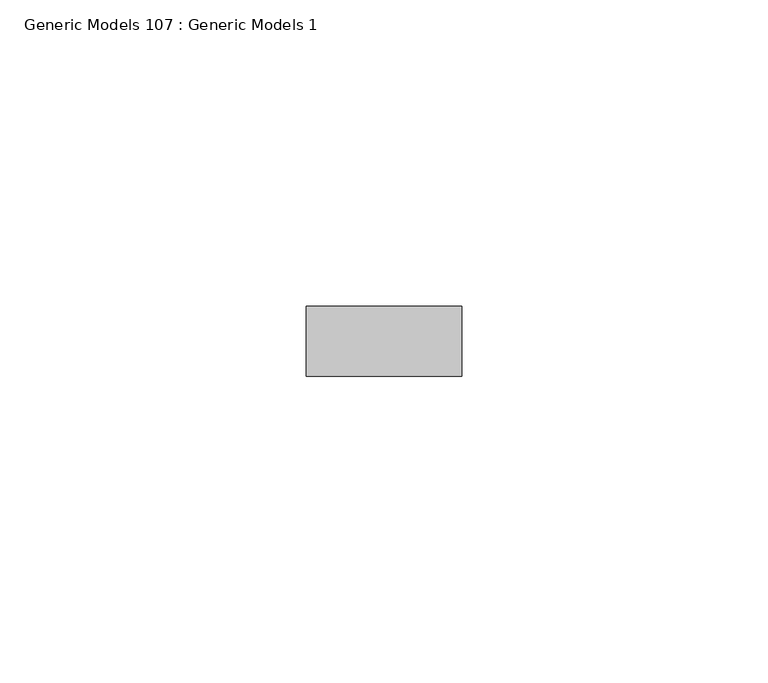
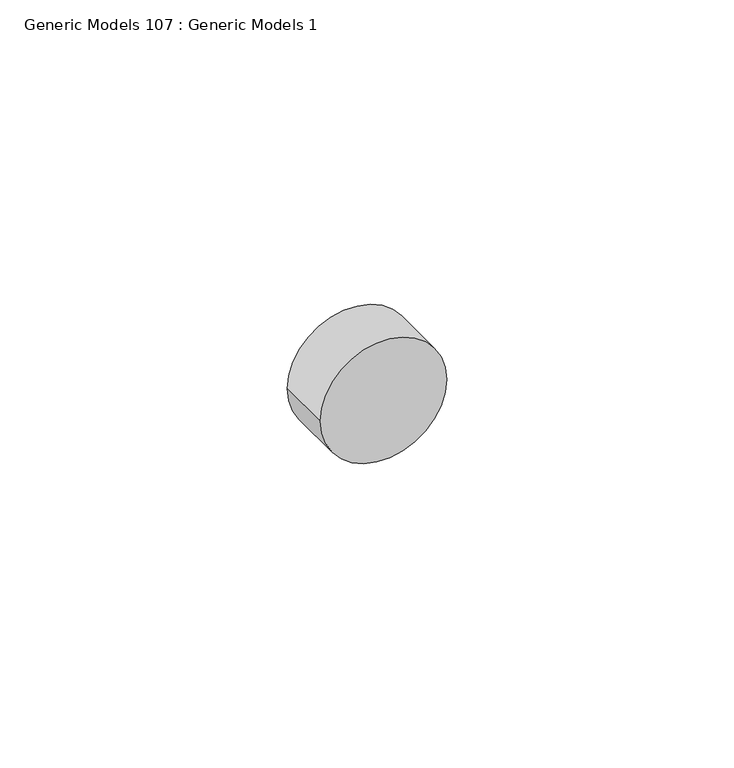
"""IFC4 building model written with IfcOpenShell, lengths in millimetres: proxy geometry, Generic Models 107 : Generic Models 1."""

from ifc_helpers import new_model, si_unit, point, frame, frame_2d, origin, place, context, project, spatial, circle_curve, trimmed, segment, composite_curve, outline, extrude, source, transform, mapped, element, save


def generic_models_107_generic_models_1_af40dd8f(model_context):
    return source(origin(), model_context, "Body", "SweptSolid", [
        extrude(outline(composite_curve([segment(trimmed(circle_curve(frame_2d((37517.3905034, 6179.9346014)), 12.7), [point((37517.3905034, 6192.6346014))], [point((37517.3905034, 6167.2346014))], False, "CARTESIAN"), True, "CONTINUOUS"), segment(trimmed(circle_curve(frame_2d((37517.3905034, 6179.9346014)), 12.7), [point((37517.3905034, 6167.2346014))], [point((37517.3905034, 6192.6346014))], False, "CARTESIAN"), True, "CONTINUOUS")], self_intersect=False)), frame((0.0, 1836.9202358, 0.0), z_axis=(0.0, 1.0, 0.0), x_axis=(0.0, 0.0, 1.0)), (0.0, 0.0, 1.0), 11.4464372),
    ])


if __name__ == "__main__":
    model = new_model("IFC4")
    model_context = context("Model", 3, world=origin())
    ifc_project = project(units=[si_unit("LENGTHUNIT", "METRE", prefix="MILLI")], contexts=[model_context])
    site = spatial("IfcSite", under=ifc_project)
    building = spatial("IfcBuilding", under=site)
    placement = place(None, origin())
    generic_models_107_generic_models_1_shape = generic_models_107_generic_models_1_af40dd8f(model_context)
    element("IfcBuildingElementProxy", 1, Name="Generic Models 107 : Generic Models 1", ObjectType="Generic Models 107 : Generic Models 1", at=placement, inside=building, context=model_context, shape_type="MappedRepresentation", body=[
        mapped(generic_models_107_generic_models_1_shape, transform((0.0, 0.0, 0.0), x_axis=(1.0, 0.0, 0.0), y_axis=(0.0, 1.0, 0.0), z_axis=(0.0, 0.0, 1.0))),
    ])
    save(model, "model.ifc")

# Revit data of these elements
# Element 1 (IfcBuildingElementProxy, "Generic Models 107 : Generic Models 1")
#   Materials on its faces: "S.S. LAG BOLT - SEE STRUCT. DWGS"
# Materials
#   "S.S. LAG BOLT - SEE STRUCT. DWGS": class "Generic", colour RGB 120 120 120, transparency 0, Cost = 0
